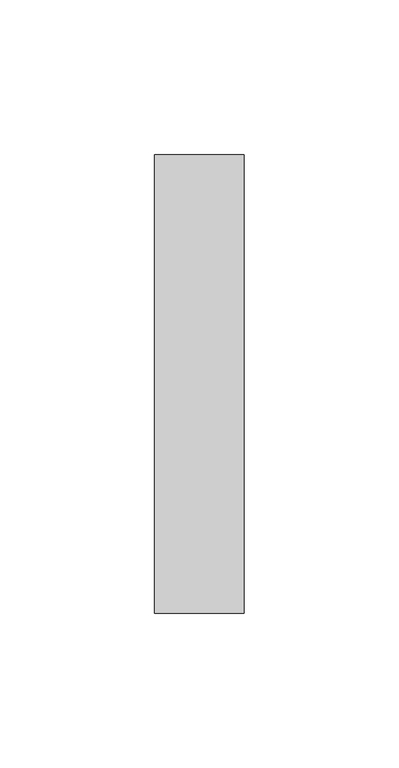
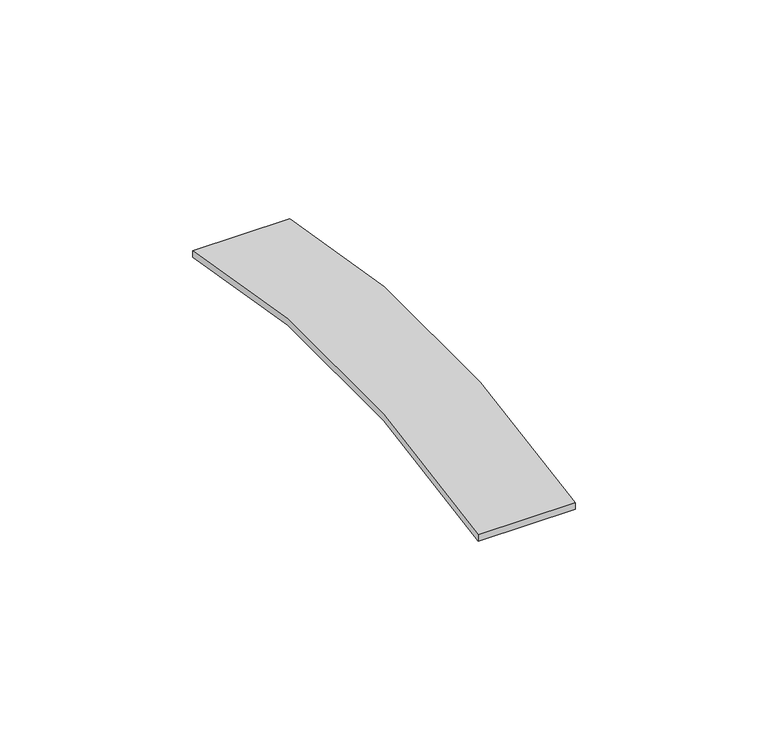
"""IFC4 building model written with IfcOpenShell, lengths in millimetres: proxy geometry, TN_ПВС 125-82_Защитная решетка : TN_ПВС 125-82_Защитная решетка."""

import ifcopenshell
import ifcopenshell.guid

model = None  # the IFC model being written
_history = None  # IfcOwnerHistory: only IFC2X3 demands one
_inside = {}  # id of a spatial element -> (the spatial element, [elements in it])
_under = {}  # id of a project, library or spatial element -> (it, [spatial elements below it])
_declared = {}  # id of a project -> (the project, [libraries it declares])
_typed = {}  # id of a type object -> (the type object, [elements of that type])
_made_of = {}  # id of a material, layer set ... -> (it, [elements and type objects made of it])


def new_model(schema):
    """Start an empty IFC model of exactly this schema.

    Asked for "IFC4X3", IfcOpenShell would pick the latest addendum, in which some entities
    have other attributes; the version numbers below select the first issue.
    IFC2X3 requires an IfcOwnerHistory on every rooted entity: one is made here for all.
    """
    global model, _history
    if schema == "IFC4X3":
        model = ifcopenshell.file(schema_version=(4, 3, 0, 0))
    else:
        model = ifcopenshell.file(schema=schema)
    _inside.clear()
    _under.clear()
    _declared.clear()
    _typed.clear()
    _made_of.clear()
    _history = None
    if model.schema == "IFC2X3":
        org = make("IfcOrganization", Name="unknown")
        user = make(
            "IfcPersonAndOrganization",
            ThePerson=make("IfcPerson", FamilyName="unknown"),
            TheOrganization=org,
        )
        app = make(
            "IfcApplication",
            ApplicationDeveloper=org,
            Version="unknown",
            ApplicationFullName="unknown",
            ApplicationIdentifier="unknown",
        )
        _history = make(
            "IfcOwnerHistory",
            OwningUser=user,
            OwningApplication=app,
            ChangeAction="ADDED",
            CreationDate=0,
        )
    return model


def make(cls, **values):
    """One entity of the class cls with the attributes given. An attribute that is None is left unset."""
    return model.create_entity(
        cls, **{name: value for name, value in values.items() if value is not None}
    )


def rooted(cls, **values):
    """An entity with a GlobalId (a new one), such as an element, a storey or a relation."""
    return make(cls, GlobalId=ifcopenshell.guid.new(), OwnerHistory=_history, **values)


def si_unit(unit_type, name, prefix=None):
    """IfcSIUnit, for example si_unit("LENGTHUNIT", "METRE", prefix="MILLI")."""
    return make("IfcSIUnit", UnitType=unit_type, Prefix=prefix, Name=name)


def assignment(units):
    """IfcUnitAssignment: the units of a project."""
    return None if units is None else make("IfcUnitAssignment", Units=units)


def point(xyz):
    """IfcCartesianPoint."""
    return None if xyz is None else make("IfcCartesianPoint", Coordinates=xyz)


def direction(xyz):
    """IfcDirection."""
    return None if xyz is None else make("IfcDirection", DirectionRatios=xyz)


def frame(location, z_axis=None, x_axis=None):
    """IfcAxis2Placement3D, a coordinate frame: its origin and axes. An axis left out is left unset."""
    return make(
        "IfcAxis2Placement3D",
        Location=point(location),
        Axis=direction(z_axis),
        RefDirection=direction(x_axis),
    )


def frame_2d(location, x_axis=None):
    """IfcAxis2Placement2D, a coordinate frame in the plane: its origin and x axis."""
    return make(
        "IfcAxis2Placement2D", Location=point(location), RefDirection=direction(x_axis)
    )


def origin():
    """The frame at (0, 0, 0) with its axes left unset."""
    return frame((0.0, 0.0, 0.0))


def place(relative_to, where):
    """IfcLocalPlacement: puts the frame where relative to a parent placement (None: the world)."""
    return make(
        "IfcLocalPlacement", PlacementRelTo=relative_to, RelativePlacement=where
    )


def context(
    kind, dimensions, precision=None, world=None, true_north=None, identifier=None
):
    """IfcGeometricRepresentationContext, for example the 3D "Model" context."""
    return make(
        "IfcGeometricRepresentationContext",
        ContextIdentifier=identifier,
        ContextType=kind,
        CoordinateSpaceDimension=dimensions,
        Precision=precision,
        WorldCoordinateSystem=world,
        TrueNorth=true_north,
    )


def project(units=None, contexts=None):
    """IfcProject with its units and contexts."""
    return rooted(
        "IfcProject",
        Name="project",
        RepresentationContexts=contexts,
        UnitsInContext=assignment(units),
    )


def spatial(cls, under=None, at=None, **own):
    """A site, building, storey or space (cls), placed at a placement, below another one or the project."""
    s = rooted(cls, ObjectPlacement=at, **own)
    if under is not None:
        _under.setdefault(under.id(), (under, []))[1].append(s)
    return s


def polyline(points):
    """IfcPolyline through the points."""
    return make("IfcPolyline", Points=[point(p) for p in points])


def circle_curve(where, radius):
    """IfcCircle in the frame where."""
    return make("IfcCircle", Position=where, Radius=radius)


def trimmed(basis, trim1, trim2, sense, master):
    """IfcTrimmedCurve: the piece of a basis curve between two trims."""
    return make(
        "IfcTrimmedCurve",
        BasisCurve=basis,
        Trim1=trim1,
        Trim2=trim2,
        SenseAgreement=sense,
        MasterRepresentation=master,
    )


def segment(curve, same_sense, transition):
    """IfcCompositeCurveSegment."""
    return make(
        "IfcCompositeCurveSegment",
        Transition=transition,
        SameSense=same_sense,
        ParentCurve=curve,
    )


def composite_curve(segments, self_intersect=None):
    """IfcCompositeCurve: segments joined end to end."""
    return make("IfcCompositeCurve", Segments=segments, SelfIntersect=self_intersect)


def outline(outer, holes=None, kind="AREA"):
    """IfcArbitraryClosedProfileDef: a profile drawn as a closed curve; with holes, ...WithVoids."""
    if holes is None:
        return make("IfcArbitraryClosedProfileDef", ProfileType=kind, OuterCurve=outer)
    return make(
        "IfcArbitraryProfileDefWithVoids",
        ProfileType=kind,
        OuterCurve=outer,
        InnerCurves=holes,
    )


def extrude(swept, where, along, depth):
    """IfcExtrudedAreaSolid: the profile swept, set in the frame where, extruded along a direction by depth."""
    return make(
        "IfcExtrudedAreaSolid",
        SweptArea=swept,
        Position=where,
        ExtrudedDirection=direction(along),
        Depth=depth,
    )


def shape(context_of_items, identifier, shape_type, items):
    """IfcShapeRepresentation: the items that make up one representation, for example the "Body"."""
    return make(
        "IfcShapeRepresentation",
        ContextOfItems=context_of_items,
        RepresentationIdentifier=identifier,
        RepresentationType=shape_type,
        Items=items,
    )


def source(mapping_origin, context_of_items, identifier, shape_type, items):
    """IfcRepresentationMap: a shape defined once, which mapped items show again and again."""
    return make(
        "IfcRepresentationMap",
        MappingOrigin=mapping_origin,
        MappedRepresentation=shape(context_of_items, identifier, shape_type, items),
    )


def transform(
    local_origin,
    x_axis=None,
    y_axis=None,
    z_axis=None,
    scale=None,
    scale2=None,
    scale3=None,
    uniform=True,
):
    """IfcCartesianTransformationOperator3D, or its non-uniform kind. x_axis, y_axis, z_axis: its Axis1, 2, 3."""
    if uniform:
        return make(
            "IfcCartesianTransformationOperator3D",
            Axis1=direction(x_axis),
            Axis2=direction(y_axis),
            LocalOrigin=point(local_origin),
            Scale=scale,
            Axis3=direction(z_axis),
        )
    return make(
        "IfcCartesianTransformationOperator3DnonUniform",
        Axis1=direction(x_axis),
        Axis2=direction(y_axis),
        LocalOrigin=point(local_origin),
        Scale=scale,
        Axis3=direction(z_axis),
        Scale2=scale2,
        Scale3=scale3,
    )


def mapped(mapping_source, mapping_target):
    """IfcMappedItem: shows the shape of a source again, moved by a transform."""
    return make(
        "IfcMappedItem", MappingSource=mapping_source, MappingTarget=mapping_target
    )


def made_of(thing, what):
    """Note that an element or type object is made of a material, layer set ...; save() writes the relation."""
    if what is not None:
        _made_of.setdefault(what.id(), (what, []))[1].append(thing)
    return thing


def element(
    cls,
    number,
    at=None,
    inside=None,
    cuts=None,
    type_object=None,
    material=None,
    context=None,
    identifier="Body",
    shape_type=None,
    held_by="IfcProductDefinitionShape",
    body=None,
    shapes=None,
    **own,
):
    """One element of the class cls, such as IfcWall. Its Tag is "e" and its number.

    at: its placement. inside: the storey or other place that contains it. cuts: it is an
    opening in that element (IfcRelVoidsElement). A single representation is given by context,
    identifier, shape_type and body (its items); several are given by shapes. held_by: the class
    of the entity that holds the representations. save() writes the other relations.
    """
    e = rooted(cls, Tag="e%d" % number, ObjectPlacement=at, **own)
    if body is not None:
        shapes = [shape(context, identifier, shape_type, body)]
    if shapes is not None:
        e.Representation = make(held_by, Representations=shapes)
    if inside is not None:
        _inside.setdefault(inside.id(), (inside, []))[1].append(e)
    if cuts is not None:
        rooted(
            "IfcRelVoidsElement", RelatingBuildingElement=cuts, RelatedOpeningElement=e
        )
    if type_object is not None:
        _typed.setdefault(type_object.id(), (type_object, []))[1].append(e)
    return made_of(e, material)


def aggregate(whole, parts):
    """IfcRelAggregates: a whole, such as a stair, and the parts it consists of."""
    return rooted("IfcRelAggregates", RelatingObject=whole, RelatedObjects=parts)


def save(model, path):
    """Write the relations noted so far, then the file.

    IfcRelAggregates (storeys below a building ...), IfcRelContainedInSpatialStructure (elements
    in a storey), IfcRelDefinesByType, IfcRelAssociatesMaterial and IfcRelDeclares: one each for
    every whole, place, type object, material and project.
    """
    for whole, parts in _under.values():
        aggregate(whole, parts)
    for where, things in _inside.values():
        rooted(
            "IfcRelContainedInSpatialStructure",
            RelatedElements=things,
            RelatingStructure=where,
        )
    for kind, things in _typed.values():
        rooted("IfcRelDefinesByType", RelatedObjects=things, RelatingType=kind)
    for what, things in _made_of.values():
        rooted("IfcRelAssociatesMaterial", RelatedObjects=things, RelatingMaterial=what)
    for by, libraries in _declared.values():
        rooted("IfcRelDeclares", RelatingContext=by, RelatedDefinitions=libraries)
    model.write(path)


def generic_models_6012d052(model_context):
    return source(origin(), model_context, "Body", "SweptSolid", [
        extrude(outline(composite_curve([segment(trimmed(circle_curve(frame_2d((0.0, -288.7046439)), 298.0), [point((74.1, -0.0644007))], [point((-74.1, -0.0644007))], True, "CARTESIAN"), True, "CONTINUOUS"), segment(polyline([(-74.1, -0.0644007), (-74.1, 2.0)]), True, "CONTINUOUS"), segment(trimmed(circle_curve(frame_2d((0.0, -288.7046439)), 300.0), [point((-74.1, 2.0))], [point((74.1, 2.0))], False, "CARTESIAN"), True, "CONTINUOUS"), segment(polyline([(74.1, 2.0), (74.1, -0.0644007)]), True, "CONTINUOUS")], self_intersect=False)), frame((0.0, 0.0, 0.0), z_axis=(1.0, 0.0, 0.0), x_axis=(0.0, 1.0, 0.0)), (0.0, 0.0, 1.0), 29.0),
    ])


if __name__ == "__main__":
    model = new_model("IFC4")
    model_context = context("Model", 3, world=origin())
    ifc_project = project(units=[si_unit("LENGTHUNIT", "METRE", prefix="MILLI")], contexts=[model_context])
    site = spatial("IfcSite", under=ifc_project)
    building = spatial("IfcBuilding", under=site)
    placement = place(None, origin())
    generic_models_shape = generic_models_6012d052(model_context)
    element("IfcBuildingElementProxy", 1, Name="TN_ПВС 125-82_Защитная решетка : TN_ПВС 125-82_Защитная решетка", ObjectType="TN_ПВС 125-82_Защитная решетка : TN_ПВС 125-82_Защитная решетка", at=placement, inside=building, context=model_context, shape_type="MappedRepresentation", body=[
        mapped(generic_models_shape, transform((0.0, 0.0, 0.0), x_axis=(1.0, 0.0, 0.0), y_axis=(0.0, 1.0, 0.0), z_axis=(0.0, 0.0, 1.0))),
    ])
    save(model, "model.ifc")

# Revit data of these elements
# Type "TN_ПВС 125-82_Защитная решетка : TN_ПВС 125-82_Защитная решетка"
#   Description = "Служит для предотвращения засора водосточной системы. Не пропускает в желоб листья и прочий крупный\r\nмусор"
#   Manufacturer = "ТехноНИКОЛЬ"
#   Model = "Комплектующие к водосточным системам"
#   URL = "https://tn-vodostok.ru/catalog/pvh/"
#   ADSK_Обозначение = "ТехноНИКОЛЬ"
#   ADSK_Наименование краткое = "Решетка"
#   ADSK_Наименование = "Защитная решетка"
#   ADSK_Масса_Текст = ""
#   ADSK_Марка = ""
#   ADSK_Код изделия = ""
#   ADSK_Завод-изготовитель = "ТехноНИКОЛЬ"
#   ADSK_Единица измерения = "п.м."
#   ADSK_Группирование = "Комплектующие к водосточным системам"
#   ADSK_URL страницы изделия = "https://tn-vodostok.ru/catalog/pvh/"
#   ADSK_URL документации изделия = "https://tn-vodostok.ru/upload/iblock/c42/c427963cb77eb5c3c51f0cfb870e9e52.pdf"
#   ADSK_Размер_Длина [instance default] = 500 mm
#   ADSK_Количество [instance default] = 0.5
#   ADSK_Материал [instance default] = TN_Пластик_Решетка_Коричневый_RAL8019
#   Default Elevation = 0
# Element 1 (IfcBuildingElementProxy, "TN_ПВС 125-82_Защитная решетка : TN_ПВС 125-82_Защитная решетка")
#   ADSK_Размер_Длина = 29 mm
#   ADSK_Количество = 0.029
#   Materials on its faces: "TN_Пластик_Решетка_Коричневый_RAL8019"
# Materials
#   "TN_Пластик_Решетка_Коричневый_RAL8019": class "Типовые", colour RGB 61 54 53, transparency 0.25, Cost = 0
